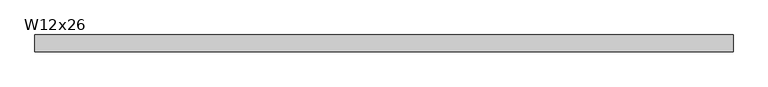
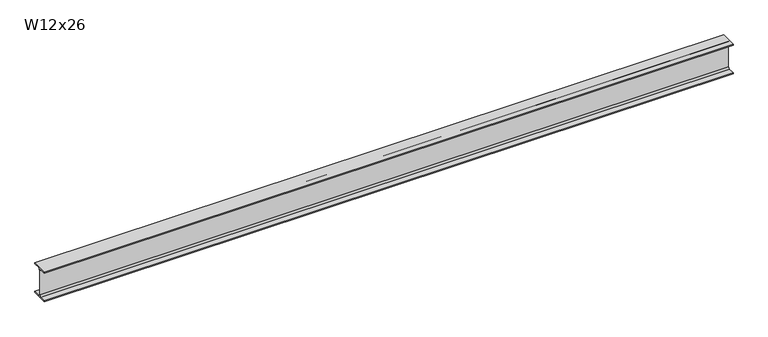
"""IFC4 building model written with IfcOpenShell, lengths in millimetres: beam geometry, RME W-Wide Flange : W12x26."""

import ifcopenshell
import ifcopenshell.guid

model = None  # the IFC model being written
_history = None  # IfcOwnerHistory: only IFC2X3 demands one
_inside = {}  # id of a spatial element -> (the spatial element, [elements in it])
_under = {}  # id of a project, library or spatial element -> (it, [spatial elements below it])
_declared = {}  # id of a project -> (the project, [libraries it declares])
_typed = {}  # id of a type object -> (the type object, [elements of that type])
_made_of = {}  # id of a material, layer set ... -> (it, [elements and type objects made of it])


def new_model(schema):
    """Start an empty IFC model of exactly this schema.

    Asked for "IFC4X3", IfcOpenShell would pick the latest addendum, in which some entities
    have other attributes; the version numbers below select the first issue.
    IFC2X3 requires an IfcOwnerHistory on every rooted entity: one is made here for all.
    """
    global model, _history
    if schema == "IFC4X3":
        model = ifcopenshell.file(schema_version=(4, 3, 0, 0))
    else:
        model = ifcopenshell.file(schema=schema)
    _inside.clear()
    _under.clear()
    _declared.clear()
    _typed.clear()
    _made_of.clear()
    _history = None
    if model.schema == "IFC2X3":
        org = make("IfcOrganization", Name="unknown")
        user = make(
            "IfcPersonAndOrganization",
            ThePerson=make("IfcPerson", FamilyName="unknown"),
            TheOrganization=org,
        )
        app = make(
            "IfcApplication",
            ApplicationDeveloper=org,
            Version="unknown",
            ApplicationFullName="unknown",
            ApplicationIdentifier="unknown",
        )
        _history = make(
            "IfcOwnerHistory",
            OwningUser=user,
            OwningApplication=app,
            ChangeAction="ADDED",
            CreationDate=0,
        )
    return model


def make(cls, **values):
    """One entity of the class cls with the attributes given. An attribute that is None is left unset."""
    return model.create_entity(
        cls, **{name: value for name, value in values.items() if value is not None}
    )


def rooted(cls, **values):
    """An entity with a GlobalId (a new one), such as an element, a storey or a relation."""
    return make(cls, GlobalId=ifcopenshell.guid.new(), OwnerHistory=_history, **values)


def si_unit(unit_type, name, prefix=None):
    """IfcSIUnit, for example si_unit("LENGTHUNIT", "METRE", prefix="MILLI")."""
    return make("IfcSIUnit", UnitType=unit_type, Prefix=prefix, Name=name)


def assignment(units):
    """IfcUnitAssignment: the units of a project."""
    return None if units is None else make("IfcUnitAssignment", Units=units)


def point(xyz):
    """IfcCartesianPoint."""
    return None if xyz is None else make("IfcCartesianPoint", Coordinates=xyz)


def direction(xyz):
    """IfcDirection."""
    return None if xyz is None else make("IfcDirection", DirectionRatios=xyz)


def frame(location, z_axis=None, x_axis=None):
    """IfcAxis2Placement3D, a coordinate frame: its origin and axes. An axis left out is left unset."""
    return make(
        "IfcAxis2Placement3D",
        Location=point(location),
        Axis=direction(z_axis),
        RefDirection=direction(x_axis),
    )


def frame_2d(location, x_axis=None):
    """IfcAxis2Placement2D, a coordinate frame in the plane: its origin and x axis."""
    return make(
        "IfcAxis2Placement2D", Location=point(location), RefDirection=direction(x_axis)
    )


def origin():
    """The frame at (0, 0, 0) with its axes left unset."""
    return frame((0.0, 0.0, 0.0))


def place(relative_to, where):
    """IfcLocalPlacement: puts the frame where relative to a parent placement (None: the world)."""
    return make(
        "IfcLocalPlacement", PlacementRelTo=relative_to, RelativePlacement=where
    )


def context(
    kind, dimensions, precision=None, world=None, true_north=None, identifier=None
):
    """IfcGeometricRepresentationContext, for example the 3D "Model" context."""
    return make(
        "IfcGeometricRepresentationContext",
        ContextIdentifier=identifier,
        ContextType=kind,
        CoordinateSpaceDimension=dimensions,
        Precision=precision,
        WorldCoordinateSystem=world,
        TrueNorth=true_north,
    )


def project(units=None, contexts=None):
    """IfcProject with its units and contexts."""
    return rooted(
        "IfcProject",
        Name="project",
        RepresentationContexts=contexts,
        UnitsInContext=assignment(units),
    )


def spatial(cls, under=None, at=None, **own):
    """A site, building, storey or space (cls), placed at a placement, below another one or the project."""
    s = rooted(cls, ObjectPlacement=at, **own)
    if under is not None:
        _under.setdefault(under.id(), (under, []))[1].append(s)
    return s


def polyline(points):
    """IfcPolyline through the points."""
    return make("IfcPolyline", Points=[point(p) for p in points])


def circle_curve(where, radius):
    """IfcCircle in the frame where."""
    return make("IfcCircle", Position=where, Radius=radius)


def trimmed(basis, trim1, trim2, sense, master):
    """IfcTrimmedCurve: the piece of a basis curve between two trims."""
    return make(
        "IfcTrimmedCurve",
        BasisCurve=basis,
        Trim1=trim1,
        Trim2=trim2,
        SenseAgreement=sense,
        MasterRepresentation=master,
    )


def segment(curve, same_sense, transition):
    """IfcCompositeCurveSegment."""
    return make(
        "IfcCompositeCurveSegment",
        Transition=transition,
        SameSense=same_sense,
        ParentCurve=curve,
    )


def composite_curve(segments, self_intersect=None):
    """IfcCompositeCurve: segments joined end to end."""
    return make("IfcCompositeCurve", Segments=segments, SelfIntersect=self_intersect)


def outline(outer, holes=None, kind="AREA"):
    """IfcArbitraryClosedProfileDef: a profile drawn as a closed curve; with holes, ...WithVoids."""
    if holes is None:
        return make("IfcArbitraryClosedProfileDef", ProfileType=kind, OuterCurve=outer)
    return make(
        "IfcArbitraryProfileDefWithVoids",
        ProfileType=kind,
        OuterCurve=outer,
        InnerCurves=holes,
    )


def extrude(swept, where, along, depth):
    """IfcExtrudedAreaSolid: the profile swept, set in the frame where, extruded along a direction by depth."""
    return make(
        "IfcExtrudedAreaSolid",
        SweptArea=swept,
        Position=where,
        ExtrudedDirection=direction(along),
        Depth=depth,
    )


def shape(context_of_items, identifier, shape_type, items):
    """IfcShapeRepresentation: the items that make up one representation, for example the "Body"."""
    return make(
        "IfcShapeRepresentation",
        ContextOfItems=context_of_items,
        RepresentationIdentifier=identifier,
        RepresentationType=shape_type,
        Items=items,
    )


def source(mapping_origin, context_of_items, identifier, shape_type, items):
    """IfcRepresentationMap: a shape defined once, which mapped items show again and again."""
    return make(
        "IfcRepresentationMap",
        MappingOrigin=mapping_origin,
        MappedRepresentation=shape(context_of_items, identifier, shape_type, items),
    )


def transform(
    local_origin,
    x_axis=None,
    y_axis=None,
    z_axis=None,
    scale=None,
    scale2=None,
    scale3=None,
    uniform=True,
):
    """IfcCartesianTransformationOperator3D, or its non-uniform kind. x_axis, y_axis, z_axis: its Axis1, 2, 3."""
    if uniform:
        return make(
            "IfcCartesianTransformationOperator3D",
            Axis1=direction(x_axis),
            Axis2=direction(y_axis),
            LocalOrigin=point(local_origin),
            Scale=scale,
            Axis3=direction(z_axis),
        )
    return make(
        "IfcCartesianTransformationOperator3DnonUniform",
        Axis1=direction(x_axis),
        Axis2=direction(y_axis),
        LocalOrigin=point(local_origin),
        Scale=scale,
        Axis3=direction(z_axis),
        Scale2=scale2,
        Scale3=scale3,
    )


def mapped(mapping_source, mapping_target):
    """IfcMappedItem: shows the shape of a source again, moved by a transform."""
    return make(
        "IfcMappedItem", MappingSource=mapping_source, MappingTarget=mapping_target
    )


def made_of(thing, what):
    """Note that an element or type object is made of a material, layer set ...; save() writes the relation."""
    if what is not None:
        _made_of.setdefault(what.id(), (what, []))[1].append(thing)
    return thing


def element(
    cls,
    number,
    at=None,
    inside=None,
    cuts=None,
    type_object=None,
    material=None,
    context=None,
    identifier="Body",
    shape_type=None,
    held_by="IfcProductDefinitionShape",
    body=None,
    shapes=None,
    **own,
):
    """One element of the class cls, such as IfcWall. Its Tag is "e" and its number.

    at: its placement. inside: the storey or other place that contains it. cuts: it is an
    opening in that element (IfcRelVoidsElement). A single representation is given by context,
    identifier, shape_type and body (its items); several are given by shapes. held_by: the class
    of the entity that holds the representations. save() writes the other relations.
    """
    e = rooted(cls, Tag="e%d" % number, ObjectPlacement=at, **own)
    if body is not None:
        shapes = [shape(context, identifier, shape_type, body)]
    if shapes is not None:
        e.Representation = make(held_by, Representations=shapes)
    if inside is not None:
        _inside.setdefault(inside.id(), (inside, []))[1].append(e)
    if cuts is not None:
        rooted(
            "IfcRelVoidsElement", RelatingBuildingElement=cuts, RelatedOpeningElement=e
        )
    if type_object is not None:
        _typed.setdefault(type_object.id(), (type_object, []))[1].append(e)
    return made_of(e, material)


def aggregate(whole, parts):
    """IfcRelAggregates: a whole, such as a stair, and the parts it consists of."""
    return rooted("IfcRelAggregates", RelatingObject=whole, RelatedObjects=parts)


def save(model, path):
    """Write the relations noted so far, then the file.

    IfcRelAggregates (storeys below a building ...), IfcRelContainedInSpatialStructure (elements
    in a storey), IfcRelDefinesByType, IfcRelAssociatesMaterial and IfcRelDeclares: one each for
    every whole, place, type object, material and project.
    """
    for whole, parts in _under.values():
        aggregate(whole, parts)
    for where, things in _inside.values():
        rooted(
            "IfcRelContainedInSpatialStructure",
            RelatedElements=things,
            RelatingStructure=where,
        )
    for kind, things in _typed.values():
        rooted("IfcRelDefinesByType", RelatedObjects=things, RelatingType=kind)
    for what, things in _made_of.values():
        rooted("IfcRelAssociatesMaterial", RelatedObjects=things, RelatingMaterial=what)
    for by, libraries in _declared.values():
        rooted("IfcRelDeclares", RelatingContext=by, RelatedDefinitions=libraries)
    model.write(path)


def w12x26_c5317eef(model_context):
    return source(origin(), model_context, "Body", "SweptSolid", [
        extrude(outline(composite_curve([segment(polyline([(82.423, -145.288), (82.423, -154.94), (-82.423, -154.94), (-82.423, -145.288), (-20.2565, -145.288)]), True, "CONTINUOUS"), segment(trimmed(circle_curve(frame_2d((-20.2565, -127.9525)), 17.3355), [point((-20.2565, -145.288))], [point((-2.921, -127.9525))], True, "CARTESIAN"), True, "CONTINUOUS"), segment(polyline([(-2.921, -127.9525), (-2.921, 127.9525)]), True, "CONTINUOUS"), segment(trimmed(circle_curve(frame_2d((-20.2565, 127.9525)), 17.3355), [point((-2.921, 127.9525))], [point((-20.2565, 145.288))], True, "CARTESIAN"), True, "CONTINUOUS"), segment(polyline([(-20.2565, 145.288), (-82.423, 145.288), (-82.423, 154.94), (82.423, 154.94), (82.423, 145.288), (20.2565, 145.288)]), True, "CONTINUOUS"), segment(trimmed(circle_curve(frame_2d((20.2565, 127.9525)), 17.3355), [point((20.2565, 145.288))], [point((2.921, 127.9525))], True, "CARTESIAN"), True, "CONTINUOUS"), segment(polyline([(2.921, 127.9525), (2.921, -127.9525)]), True, "CONTINUOUS"), segment(trimmed(circle_curve(frame_2d((20.2565, -127.9525)), 17.3355), [point((2.921, -127.9525))], [point((20.2565, -145.288))], True, "CARTESIAN"), True, "CONTINUOUS"), segment(polyline([(20.2565, -145.288), (82.423, -145.288)]), True, "CONTINUOUS")], self_intersect=False)), frame((-3575.0499994, 0.0, 0.0), z_axis=(1.0, 0.0, 0.0), x_axis=(0.0, 1.0, 0.0)), (0.0, 0.0, 1.0), 6857.9999994),
    ])


if __name__ == "__main__":
    model = new_model("IFC4")
    model_context = context("Model", 3, world=origin())
    ifc_project = project(units=[si_unit("LENGTHUNIT", "METRE", prefix="MILLI")], contexts=[model_context])
    site = spatial("IfcSite", under=ifc_project)
    building = spatial("IfcBuilding", under=site)
    placement = place(None, origin())
    w12x26_shape = w12x26_c5317eef(model_context)
    element("IfcBeam", 1, ObjectType="RME W-Wide Flange : W12x26", at=placement, inside=building, context=model_context, shape_type="MappedRepresentation", body=[
        mapped(w12x26_shape, transform((0.0, 0.0, 0.0), x_axis=(1.0, 0.0, 0.0), y_axis=(0.0, 1.0, 0.0), z_axis=(0.0, 0.0, 1.0))),
    ])
    save(model, "model.ifc")

# Revit data of these elements
# Type "RME W-Wide Flange : W12x26"
#   WELD P [instance default] = ""
#   WELD LE [instance default] = ""
#   WELD D [instance default] = ""
#   TOP SECTION SIZE [instance default] = ""
#   TOP SECTION LENGTH [instance default] = ""
#   REMARKS [instance default] = ""
#   REINF TYPE [instance default] = ""
#   Nominal Size = "W24"
#   End Bearing Capacity [instance default] = ""
#   BOT SECTION SIZE [instance default] = ""
#   BOT SECTION LENGTH [instance default] = ""
#   Assembly Code = "B10"
#   W = 26
#   Start Extension Calculation [instance default] = 10' - 0"
#   Start Extension [instance default] = -0' - 0 1/2"
#   End Extension Calculation [instance default] = 10' - 0"
#   End Extension [instance default] = -0' - 0 1/2"
#   Length [instance default] = 5' - 0"
#   bf = 0' - 6.49"
#   d = 1' - 0.2"
#   k = 0' - 1 1/16"
#   k2 = 0' - 0.6825"
#   tf = 0' - 0.38"
#   tw = 0' - 0.23"
#   A = 0.053125 SF
#   Structural Material [instance default] = Metal - Steel - ASTM A992
# Element 1 (IfcBeam, "RME W-Wide Flange : W12x26")
#   Length = 23' - 6 1/2"
#   Materials on its faces: "Metal - Steel - ASTM A992"
# Materials
#   "Metal - Steel - ASTM A992": class "Metal", colour RGB 255 128 0, transparency 0
